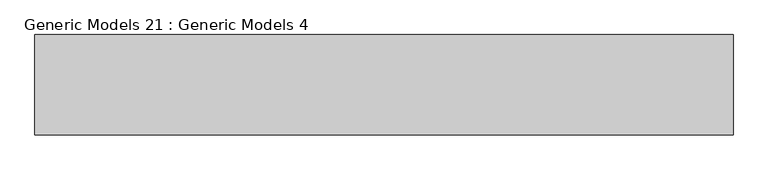
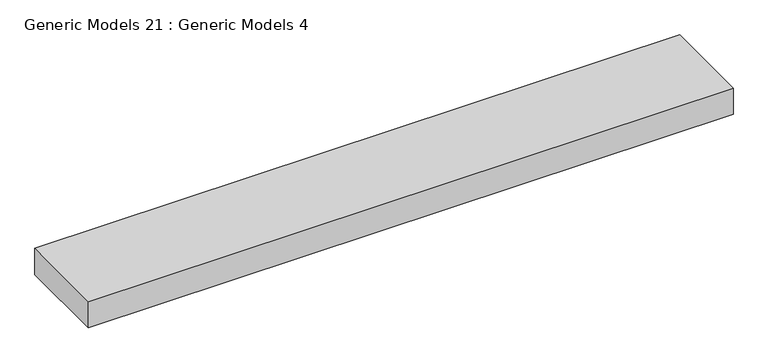
"""IFC4 building model written with IfcOpenShell, lengths in millimetres: proxy geometry, Generic Models 21 : Generic Models 4."""

from ifc_helpers import new_model, si_unit, frame, origin, place, context, project, spatial, polyline, outline, extrude, source, transform, mapped, element, save


def generic_models_21_generic_models_4_ff154e53(model_context):
    return source(origin(), model_context, "Body", "SweptSolid", [
        extrude(outline(polyline([(8386.8578684, -6119.2029588), (8386.8578684, -7007.9785995), (2196.9263704, -7007.9785995), (2196.9263704, -6119.2029588), (8386.8578684, -6119.2029588)])), frame((0.0, 0.0, 126489.9460277), z_axis=(0.0, 0.0, 1.0), x_axis=(1.0, 0.0, 0.0)), (0.0, 0.0, 1.0), 266.7),
    ])


if __name__ == "__main__":
    model = new_model("IFC4")
    model_context = context("Model", 3, world=origin())
    ifc_project = project(units=[si_unit("LENGTHUNIT", "METRE", prefix="MILLI")], contexts=[model_context])
    site = spatial("IfcSite", under=ifc_project)
    building = spatial("IfcBuilding", under=site)
    placement = place(None, origin())
    generic_models_21_generic_models_4_shape = generic_models_21_generic_models_4_ff154e53(model_context)
    element("IfcBuildingElementProxy", 1, Name="Generic Models 21 : Generic Models 4", ObjectType="Generic Models 21 : Generic Models 4", at=placement, inside=building, context=model_context, shape_type="MappedRepresentation", body=[
        mapped(generic_models_21_generic_models_4_shape, transform((0.0, 0.0, 0.0), x_axis=(1.0, 0.0, 0.0), y_axis=(0.0, 1.0, 0.0), z_axis=(0.0, 0.0, 1.0))),
    ])
    save(model, "model.ifc")

# Revit data of these elements
# Element 1 (IfcBuildingElementProxy, "Generic Models 21 : Generic Models 4")
#   Materials on its faces: "_BATT INSUL. (R-FACTOR = R38 MIN) OVER CLASS II VAPOR RETARDER(TOWARD INTERIOR)"
# Materials
#   "_BATT INSUL. (R-FACTOR = R38 MIN) OVER CLASS II VAPOR RETARDER(TOWARD INTERIOR)": class "Generic", colour RGB 227 210 251, transparency 0, Cost = 0
